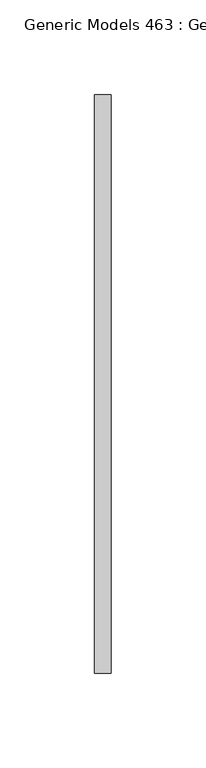
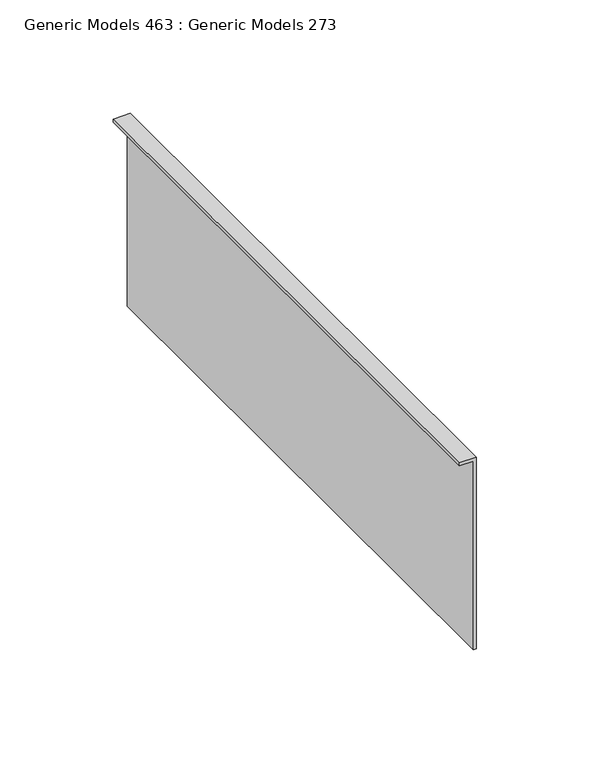
"""IFC4 building model written with IfcOpenShell, lengths in millimetres: proxy geometry, Generic Models 463 : Generic Models 273."""

import ifcopenshell
import ifcopenshell.guid

model = None  # the IFC model being written
_history = None  # IfcOwnerHistory: only IFC2X3 demands one
_inside = {}  # id of a spatial element -> (the spatial element, [elements in it])
_under = {}  # id of a project, library or spatial element -> (it, [spatial elements below it])
_declared = {}  # id of a project -> (the project, [libraries it declares])
_typed = {}  # id of a type object -> (the type object, [elements of that type])
_made_of = {}  # id of a material, layer set ... -> (it, [elements and type objects made of it])


def new_model(schema):
    """Start an empty IFC model of exactly this schema.

    Asked for "IFC4X3", IfcOpenShell would pick the latest addendum, in which some entities
    have other attributes; the version numbers below select the first issue.
    IFC2X3 requires an IfcOwnerHistory on every rooted entity: one is made here for all.
    """
    global model, _history
    if schema == "IFC4X3":
        model = ifcopenshell.file(schema_version=(4, 3, 0, 0))
    else:
        model = ifcopenshell.file(schema=schema)
    _inside.clear()
    _under.clear()
    _declared.clear()
    _typed.clear()
    _made_of.clear()
    _history = None
    if model.schema == "IFC2X3":
        org = make("IfcOrganization", Name="unknown")
        user = make(
            "IfcPersonAndOrganization",
            ThePerson=make("IfcPerson", FamilyName="unknown"),
            TheOrganization=org,
        )
        app = make(
            "IfcApplication",
            ApplicationDeveloper=org,
            Version="unknown",
            ApplicationFullName="unknown",
            ApplicationIdentifier="unknown",
        )
        _history = make(
            "IfcOwnerHistory",
            OwningUser=user,
            OwningApplication=app,
            ChangeAction="ADDED",
            CreationDate=0,
        )
    return model


def make(cls, **values):
    """One entity of the class cls with the attributes given. An attribute that is None is left unset."""
    return model.create_entity(
        cls, **{name: value for name, value in values.items() if value is not None}
    )


def rooted(cls, **values):
    """An entity with a GlobalId (a new one), such as an element, a storey or a relation."""
    return make(cls, GlobalId=ifcopenshell.guid.new(), OwnerHistory=_history, **values)


def si_unit(unit_type, name, prefix=None):
    """IfcSIUnit, for example si_unit("LENGTHUNIT", "METRE", prefix="MILLI")."""
    return make("IfcSIUnit", UnitType=unit_type, Prefix=prefix, Name=name)


def assignment(units):
    """IfcUnitAssignment: the units of a project."""
    return None if units is None else make("IfcUnitAssignment", Units=units)


def point(xyz):
    """IfcCartesianPoint."""
    return None if xyz is None else make("IfcCartesianPoint", Coordinates=xyz)


def direction(xyz):
    """IfcDirection."""
    return None if xyz is None else make("IfcDirection", DirectionRatios=xyz)


def frame(location, z_axis=None, x_axis=None):
    """IfcAxis2Placement3D, a coordinate frame: its origin and axes. An axis left out is left unset."""
    return make(
        "IfcAxis2Placement3D",
        Location=point(location),
        Axis=direction(z_axis),
        RefDirection=direction(x_axis),
    )


def origin():
    """The frame at (0, 0, 0) with its axes left unset."""
    return frame((0.0, 0.0, 0.0))


def place(relative_to, where):
    """IfcLocalPlacement: puts the frame where relative to a parent placement (None: the world)."""
    return make(
        "IfcLocalPlacement", PlacementRelTo=relative_to, RelativePlacement=where
    )


def context(
    kind, dimensions, precision=None, world=None, true_north=None, identifier=None
):
    """IfcGeometricRepresentationContext, for example the 3D "Model" context."""
    return make(
        "IfcGeometricRepresentationContext",
        ContextIdentifier=identifier,
        ContextType=kind,
        CoordinateSpaceDimension=dimensions,
        Precision=precision,
        WorldCoordinateSystem=world,
        TrueNorth=true_north,
    )


def project(units=None, contexts=None):
    """IfcProject with its units and contexts."""
    return rooted(
        "IfcProject",
        Name="project",
        RepresentationContexts=contexts,
        UnitsInContext=assignment(units),
    )


def spatial(cls, under=None, at=None, **own):
    """A site, building, storey or space (cls), placed at a placement, below another one or the project."""
    s = rooted(cls, ObjectPlacement=at, **own)
    if under is not None:
        _under.setdefault(under.id(), (under, []))[1].append(s)
    return s


def polyline(points):
    """IfcPolyline through the points."""
    return make("IfcPolyline", Points=[point(p) for p in points])


def outline(outer, holes=None, kind="AREA"):
    """IfcArbitraryClosedProfileDef: a profile drawn as a closed curve; with holes, ...WithVoids."""
    if holes is None:
        return make("IfcArbitraryClosedProfileDef", ProfileType=kind, OuterCurve=outer)
    return make(
        "IfcArbitraryProfileDefWithVoids",
        ProfileType=kind,
        OuterCurve=outer,
        InnerCurves=holes,
    )


def extrude(swept, where, along, depth):
    """IfcExtrudedAreaSolid: the profile swept, set in the frame where, extruded along a direction by depth."""
    return make(
        "IfcExtrudedAreaSolid",
        SweptArea=swept,
        Position=where,
        ExtrudedDirection=direction(along),
        Depth=depth,
    )


def shape(context_of_items, identifier, shape_type, items):
    """IfcShapeRepresentation: the items that make up one representation, for example the "Body"."""
    return make(
        "IfcShapeRepresentation",
        ContextOfItems=context_of_items,
        RepresentationIdentifier=identifier,
        RepresentationType=shape_type,
        Items=items,
    )


def source(mapping_origin, context_of_items, identifier, shape_type, items):
    """IfcRepresentationMap: a shape defined once, which mapped items show again and again."""
    return make(
        "IfcRepresentationMap",
        MappingOrigin=mapping_origin,
        MappedRepresentation=shape(context_of_items, identifier, shape_type, items),
    )


def transform(
    local_origin,
    x_axis=None,
    y_axis=None,
    z_axis=None,
    scale=None,
    scale2=None,
    scale3=None,
    uniform=True,
):
    """IfcCartesianTransformationOperator3D, or its non-uniform kind. x_axis, y_axis, z_axis: its Axis1, 2, 3."""
    if uniform:
        return make(
            "IfcCartesianTransformationOperator3D",
            Axis1=direction(x_axis),
            Axis2=direction(y_axis),
            LocalOrigin=point(local_origin),
            Scale=scale,
            Axis3=direction(z_axis),
        )
    return make(
        "IfcCartesianTransformationOperator3DnonUniform",
        Axis1=direction(x_axis),
        Axis2=direction(y_axis),
        LocalOrigin=point(local_origin),
        Scale=scale,
        Axis3=direction(z_axis),
        Scale2=scale2,
        Scale3=scale3,
    )


def mapped(mapping_source, mapping_target):
    """IfcMappedItem: shows the shape of a source again, moved by a transform."""
    return make(
        "IfcMappedItem", MappingSource=mapping_source, MappingTarget=mapping_target
    )


def made_of(thing, what):
    """Note that an element or type object is made of a material, layer set ...; save() writes the relation."""
    if what is not None:
        _made_of.setdefault(what.id(), (what, []))[1].append(thing)
    return thing


def element(
    cls,
    number,
    at=None,
    inside=None,
    cuts=None,
    type_object=None,
    material=None,
    context=None,
    identifier="Body",
    shape_type=None,
    held_by="IfcProductDefinitionShape",
    body=None,
    shapes=None,
    **own,
):
    """One element of the class cls, such as IfcWall. Its Tag is "e" and its number.

    at: its placement. inside: the storey or other place that contains it. cuts: it is an
    opening in that element (IfcRelVoidsElement). A single representation is given by context,
    identifier, shape_type and body (its items); several are given by shapes. held_by: the class
    of the entity that holds the representations. save() writes the other relations.
    """
    e = rooted(cls, Tag="e%d" % number, ObjectPlacement=at, **own)
    if body is not None:
        shapes = [shape(context, identifier, shape_type, body)]
    if shapes is not None:
        e.Representation = make(held_by, Representations=shapes)
    if inside is not None:
        _inside.setdefault(inside.id(), (inside, []))[1].append(e)
    if cuts is not None:
        rooted(
            "IfcRelVoidsElement", RelatingBuildingElement=cuts, RelatedOpeningElement=e
        )
    if type_object is not None:
        _typed.setdefault(type_object.id(), (type_object, []))[1].append(e)
    return made_of(e, material)


def aggregate(whole, parts):
    """IfcRelAggregates: a whole, such as a stair, and the parts it consists of."""
    return rooted("IfcRelAggregates", RelatingObject=whole, RelatedObjects=parts)


def save(model, path):
    """Write the relations noted so far, then the file.

    IfcRelAggregates (storeys below a building ...), IfcRelContainedInSpatialStructure (elements
    in a storey), IfcRelDefinesByType, IfcRelAssociatesMaterial and IfcRelDeclares: one each for
    every whole, place, type object, material and project.
    """
    for whole, parts in _under.values():
        aggregate(whole, parts)
    for where, things in _inside.values():
        rooted(
            "IfcRelContainedInSpatialStructure",
            RelatedElements=things,
            RelatingStructure=where,
        )
    for kind, things in _typed.values():
        rooted("IfcRelDefinesByType", RelatedObjects=things, RelatingType=kind)
    for what, things in _made_of.values():
        rooted("IfcRelAssociatesMaterial", RelatedObjects=things, RelatingMaterial=what)
    for by, libraries in _declared.values():
        rooted("IfcRelDeclares", RelatingContext=by, RelatedDefinitions=libraries)
    model.write(path)


def generic_models_463_generic_models_273_ee130d9c(model_context):
    return source(origin(), model_context, "Body", "SweptSolid", [
        extrude(outline(polyline([(123479.2434678, 1666.6695929), (123479.2434678, 1658.0612048), (123477.6559678, 1658.0612048), (123477.6559678, 1665.0820929), (123376.0559678, 1665.0820929), (123376.0559678, 1666.6695929), (123479.2434678, 1666.6695929)])), frame((0.0, 4260.0872686, 0.0), z_axis=(0.0, 1.0, 0.0), x_axis=(0.0, 0.0, 1.0)), (0.0, 0.0, 1.0), 304.8),
    ])


if __name__ == "__main__":
    model = new_model("IFC4")
    model_context = context("Model", 3, world=origin())
    ifc_project = project(units=[si_unit("LENGTHUNIT", "METRE", prefix="MILLI")], contexts=[model_context])
    site = spatial("IfcSite", under=ifc_project)
    building = spatial("IfcBuilding", under=site)
    placement = place(None, origin())
    generic_models_463_generic_models_273_shape = generic_models_463_generic_models_273_ee130d9c(model_context)
    element("IfcBuildingElementProxy", 1, Name="Generic Models 463 : Generic Models 273", ObjectType="Generic Models 463 : Generic Models 273", at=placement, inside=building, context=model_context, shape_type="MappedRepresentation", body=[
        mapped(generic_models_463_generic_models_273_shape, transform((0.0, 0.0, 0.0), x_axis=(1.0, 0.0, 0.0), y_axis=(0.0, 1.0, 0.0), z_axis=(0.0, 0.0, 1.0))),
    ])
    save(model, "model.ifc")

# Revit data of these elements
# Element 1 (IfcBuildingElementProxy, "Generic Models 463 : Generic Models 273")
#   Materials on its faces: "_ALUM. MULLION CAP BY WINDOW MANUFACTURER (COLOR T.B.D)"
# Materials
#   "_ALUM. MULLION CAP BY WINDOW MANUFACTURER (COLOR T.B.D)": class "Metal", colour RGB 199 199 199, transparency 0, Description = "Structural steel 50ksi", Cost = 0
